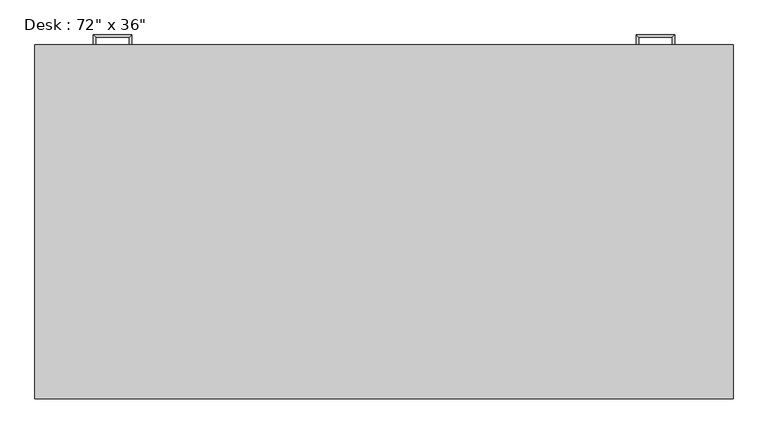
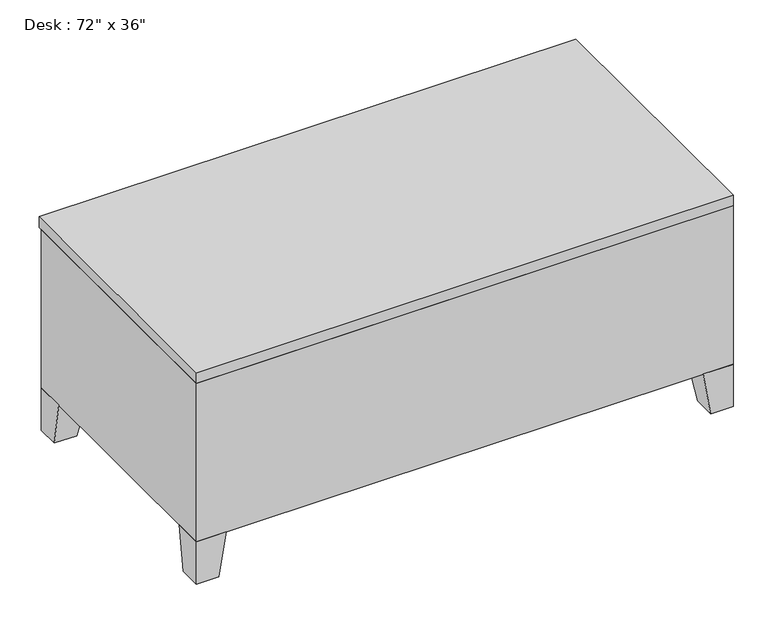
"""IFC4 building model written with IfcOpenShell, lengths in millimetres: furniture geometry."""

import ifcopenshell
import ifcopenshell.guid

model = None  # the IFC model being written
_history = None  # IfcOwnerHistory: only IFC2X3 demands one
_inside = {}  # id of a spatial element -> (the spatial element, [elements in it])
_under = {}  # id of a project, library or spatial element -> (it, [spatial elements below it])
_declared = {}  # id of a project -> (the project, [libraries it declares])
_typed = {}  # id of a type object -> (the type object, [elements of that type])
_made_of = {}  # id of a material, layer set ... -> (it, [elements and type objects made of it])


def new_model(schema):
    """Start an empty IFC model of exactly this schema.

    Asked for "IFC4X3", IfcOpenShell would pick the latest addendum, in which some entities
    have other attributes; the version numbers below select the first issue.
    IFC2X3 requires an IfcOwnerHistory on every rooted entity: one is made here for all.
    """
    global model, _history
    if schema == "IFC4X3":
        model = ifcopenshell.file(schema_version=(4, 3, 0, 0))
    else:
        model = ifcopenshell.file(schema=schema)
    _inside.clear()
    _under.clear()
    _declared.clear()
    _typed.clear()
    _made_of.clear()
    _history = None
    if model.schema == "IFC2X3":
        org = make("IfcOrganization", Name="unknown")
        user = make(
            "IfcPersonAndOrganization",
            ThePerson=make("IfcPerson", FamilyName="unknown"),
            TheOrganization=org,
        )
        app = make(
            "IfcApplication",
            ApplicationDeveloper=org,
            Version="unknown",
            ApplicationFullName="unknown",
            ApplicationIdentifier="unknown",
        )
        _history = make(
            "IfcOwnerHistory",
            OwningUser=user,
            OwningApplication=app,
            ChangeAction="ADDED",
            CreationDate=0,
        )
    return model


def make(cls, **values):
    """One entity of the class cls with the attributes given. An attribute that is None is left unset."""
    return model.create_entity(
        cls, **{name: value for name, value in values.items() if value is not None}
    )


def rooted(cls, **values):
    """An entity with a GlobalId (a new one), such as an element, a storey or a relation."""
    return make(cls, GlobalId=ifcopenshell.guid.new(), OwnerHistory=_history, **values)


def si_unit(unit_type, name, prefix=None):
    """IfcSIUnit, for example si_unit("LENGTHUNIT", "METRE", prefix="MILLI")."""
    return make("IfcSIUnit", UnitType=unit_type, Prefix=prefix, Name=name)


def assignment(units):
    """IfcUnitAssignment: the units of a project."""
    return None if units is None else make("IfcUnitAssignment", Units=units)


def point(xyz):
    """IfcCartesianPoint."""
    return None if xyz is None else make("IfcCartesianPoint", Coordinates=xyz)


def direction(xyz):
    """IfcDirection."""
    return None if xyz is None else make("IfcDirection", DirectionRatios=xyz)


def frame(location, z_axis=None, x_axis=None):
    """IfcAxis2Placement3D, a coordinate frame: its origin and axes. An axis left out is left unset."""
    return make(
        "IfcAxis2Placement3D",
        Location=point(location),
        Axis=direction(z_axis),
        RefDirection=direction(x_axis),
    )


def origin():
    """The frame at (0, 0, 0) with its axes left unset."""
    return frame((0.0, 0.0, 0.0))


def place(relative_to, where):
    """IfcLocalPlacement: puts the frame where relative to a parent placement (None: the world)."""
    return make(
        "IfcLocalPlacement", PlacementRelTo=relative_to, RelativePlacement=where
    )


def context(
    kind, dimensions, precision=None, world=None, true_north=None, identifier=None
):
    """IfcGeometricRepresentationContext, for example the 3D "Model" context."""
    return make(
        "IfcGeometricRepresentationContext",
        ContextIdentifier=identifier,
        ContextType=kind,
        CoordinateSpaceDimension=dimensions,
        Precision=precision,
        WorldCoordinateSystem=world,
        TrueNorth=true_north,
    )


def project(units=None, contexts=None):
    """IfcProject with its units and contexts."""
    return rooted(
        "IfcProject",
        Name="project",
        RepresentationContexts=contexts,
        UnitsInContext=assignment(units),
    )


def spatial(cls, under=None, at=None, **own):
    """A site, building, storey or space (cls), placed at a placement, below another one or the project."""
    s = rooted(cls, ObjectPlacement=at, **own)
    if under is not None:
        _under.setdefault(under.id(), (under, []))[1].append(s)
    return s


def polyline(points):
    """IfcPolyline through the points."""
    return make("IfcPolyline", Points=[point(p) for p in points])


def outline(outer, holes=None, kind="AREA"):
    """IfcArbitraryClosedProfileDef: a profile drawn as a closed curve; with holes, ...WithVoids."""
    if holes is None:
        return make("IfcArbitraryClosedProfileDef", ProfileType=kind, OuterCurve=outer)
    return make(
        "IfcArbitraryProfileDefWithVoids",
        ProfileType=kind,
        OuterCurve=outer,
        InnerCurves=holes,
    )


def extrude(swept, where, along, depth):
    """IfcExtrudedAreaSolid: the profile swept, set in the frame where, extruded along a direction by depth."""
    return make(
        "IfcExtrudedAreaSolid",
        SweptArea=swept,
        Position=where,
        ExtrudedDirection=direction(along),
        Depth=depth,
    )


def faces_of(points, faces, orient=None, outer=None):
    """IfcFace entities. A face is a list of loops; a loop is a list of indices into points, from 0.

    orient and outer hold one flag for each loop. By default every Orientation is true, the
    first loop of a face is its IfcFaceOuterBound and the others are IfcFaceBound.
    """
    made = []
    for i, loops in enumerate(faces):
        bounds = []
        for j, loop in enumerate(loops):
            is_outer = j == 0 if outer is None else outer[i][j]
            bounds.append(
                make(
                    "IfcFaceOuterBound" if is_outer else "IfcFaceBound",
                    Bound=make("IfcPolyLoop", Polygon=[points[k] for k in loop]),
                    Orientation=True if orient is None else orient[i][j],
                )
            )
        made.append(make("IfcFace", Bounds=bounds))
    return made


def faceted_brep(points, faces, orient=None, outer=None, voids=None):
    """IfcFacetedBrep: a solid bounded by flat faces; with voids (closed shells), ...WithVoids."""
    shared = [point(p) for p in points]
    hull = make("IfcClosedShell", CfsFaces=faces_of(shared, faces, orient, outer))
    if voids is None:
        return make("IfcFacetedBrep", Outer=hull)
    return make(
        "IfcFacetedBrepWithVoids",
        Outer=hull,
        Voids=[
            make(cls, CfsFaces=faces_of(shared, fs, o, b)) for cls, fs, o, b in voids
        ],
    )


def shape(context_of_items, identifier, shape_type, items):
    """IfcShapeRepresentation: the items that make up one representation, for example the "Body"."""
    return make(
        "IfcShapeRepresentation",
        ContextOfItems=context_of_items,
        RepresentationIdentifier=identifier,
        RepresentationType=shape_type,
        Items=items,
    )


def source(mapping_origin, context_of_items, identifier, shape_type, items):
    """IfcRepresentationMap: a shape defined once, which mapped items show again and again."""
    return make(
        "IfcRepresentationMap",
        MappingOrigin=mapping_origin,
        MappedRepresentation=shape(context_of_items, identifier, shape_type, items),
    )


def transform(
    local_origin,
    x_axis=None,
    y_axis=None,
    z_axis=None,
    scale=None,
    scale2=None,
    scale3=None,
    uniform=True,
):
    """IfcCartesianTransformationOperator3D, or its non-uniform kind. x_axis, y_axis, z_axis: its Axis1, 2, 3."""
    if uniform:
        return make(
            "IfcCartesianTransformationOperator3D",
            Axis1=direction(x_axis),
            Axis2=direction(y_axis),
            LocalOrigin=point(local_origin),
            Scale=scale,
            Axis3=direction(z_axis),
        )
    return make(
        "IfcCartesianTransformationOperator3DnonUniform",
        Axis1=direction(x_axis),
        Axis2=direction(y_axis),
        LocalOrigin=point(local_origin),
        Scale=scale,
        Axis3=direction(z_axis),
        Scale2=scale2,
        Scale3=scale3,
    )


def mapped(mapping_source, mapping_target):
    """IfcMappedItem: shows the shape of a source again, moved by a transform."""
    return make(
        "IfcMappedItem", MappingSource=mapping_source, MappingTarget=mapping_target
    )


def made_of(thing, what):
    """Note that an element or type object is made of a material, layer set ...; save() writes the relation."""
    if what is not None:
        _made_of.setdefault(what.id(), (what, []))[1].append(thing)
    return thing


def element(
    cls,
    number,
    at=None,
    inside=None,
    cuts=None,
    type_object=None,
    material=None,
    context=None,
    identifier="Body",
    shape_type=None,
    held_by="IfcProductDefinitionShape",
    body=None,
    shapes=None,
    **own,
):
    """One element of the class cls, such as IfcWall. Its Tag is "e" and its number.

    at: its placement. inside: the storey or other place that contains it. cuts: it is an
    opening in that element (IfcRelVoidsElement). A single representation is given by context,
    identifier, shape_type and body (its items); several are given by shapes. held_by: the class
    of the entity that holds the representations. save() writes the other relations.
    """
    e = rooted(cls, Tag="e%d" % number, ObjectPlacement=at, **own)
    if body is not None:
        shapes = [shape(context, identifier, shape_type, body)]
    if shapes is not None:
        e.Representation = make(held_by, Representations=shapes)
    if inside is not None:
        _inside.setdefault(inside.id(), (inside, []))[1].append(e)
    if cuts is not None:
        rooted(
            "IfcRelVoidsElement", RelatingBuildingElement=cuts, RelatedOpeningElement=e
        )
    if type_object is not None:
        _typed.setdefault(type_object.id(), (type_object, []))[1].append(e)
    return made_of(e, material)


def aggregate(whole, parts):
    """IfcRelAggregates: a whole, such as a stair, and the parts it consists of."""
    return rooted("IfcRelAggregates", RelatingObject=whole, RelatedObjects=parts)


def save(model, path):
    """Write the relations noted so far, then the file.

    IfcRelAggregates (storeys below a building ...), IfcRelContainedInSpatialStructure (elements
    in a storey), IfcRelDefinesByType, IfcRelAssociatesMaterial and IfcRelDeclares: one each for
    every whole, place, type object, material and project.
    """
    for whole, parts in _under.values():
        aggregate(whole, parts)
    for where, things in _inside.values():
        rooted(
            "IfcRelContainedInSpatialStructure",
            RelatedElements=things,
            RelatingStructure=where,
        )
    for kind, things in _typed.values():
        rooted("IfcRelDefinesByType", RelatedObjects=things, RelatingType=kind)
    for what, things in _made_of.values():
        rooted("IfcRelAssociatesMaterial", RelatedObjects=things, RelatingMaterial=what)
    for by, libraries in _declared.values():
        rooted("IfcRelDeclares", RelatingContext=by, RelatedDefinitions=libraries)
    model.write(path)


def furniture_65204735(model_context):
    return source(origin(), model_context, "Body", "SolidModel", [
        extrude(outline(polyline([(-133.35, 76.2), (-133.35, 88.9), (234.95, 88.9), (234.95, 76.2), (-133.35, 76.2)])), frame((0.0, 0.0, 603.25), z_axis=(0.0, 0.0, 1.0), x_axis=(1.0, 0.0, 0.0)), (0.0, 0.0, 1.0), 101.6),
        extrude(outline(polyline([(-133.35, 76.2), (-133.35, 88.9), (234.95, 88.9), (234.95, 76.2), (-133.35, 76.2)])), frame((0.0, 0.0, 171.45), z_axis=(0.0, 0.0, 1.0), x_axis=(1.0, 0.0, 0.0)), (0.0, 0.0, 1.0), 412.75),
        extrude(outline(polyline([(1289.05, 76.2), (1289.05, 88.9), (1657.35, 88.9), (1657.35, 76.2), (1289.05, 76.2)])), frame((0.0, 0.0, 603.25), z_axis=(0.0, 0.0, 1.0), x_axis=(1.0, 0.0, 0.0)), (0.0, 0.0, 1.0), 101.6),
        extrude(outline(polyline([(1289.05, 76.2), (1289.05, 88.9), (1657.35, 88.9), (1657.35, 76.2), (1289.05, 76.2)])), frame((0.0, 0.0, 171.45), z_axis=(0.0, 0.0, 1.0), x_axis=(1.0, 0.0, 0.0)), (0.0, 0.0, 1.0), 171.45),
        extrude(outline(polyline([(1289.05, 76.2), (1289.05, 88.9), (1657.35, 88.9), (1657.35, 76.2), (1289.05, 76.2)])), frame((0.0, 0.0, 482.6), z_axis=(0.0, 0.0, 1.0), x_axis=(1.0, 0.0, 0.0)), (0.0, 0.0, 1.0), 101.6),
        extrude(outline(polyline([(1289.05, 76.2), (1289.05, 88.9), (1657.35, 88.9), (1657.35, 76.2), (1289.05, 76.2)])), frame((0.0, 0.0, 361.95), z_axis=(0.0, 0.0, 1.0), x_axis=(1.0, 0.0, 0.0)), (0.0, 0.0, 1.0), 101.6),
        faceted_brep([(-50.8, 76.2, 152.4), (-152.4, 76.2, 152.4), (-152.4, -25.4, 152.4), (-50.8, -25.4, 152.4), (-76.2, 76.2, 0.0), (-76.2, 0.0, 0.0), (-152.4, 0.0, 0.0), (-152.4, 76.2, 0.0)], [[[0, 1, 2, 3]], [[4, 5, 6, 7]], [[4, 0, 3, 5]], [[5, 3, 2, 6]], [[6, 2, 1, 7]], [[7, 1, 0, 4]]]),
        faceted_brep([(-50.8, -838.2, 152.4), (-50.8, -736.6, 152.4), (-152.4, -736.6, 152.4), (-152.4, -838.2, 152.4), (-76.2, -838.2, 0.0), (-152.4, -838.2, 0.0), (-152.4, -762.0, 0.0), (-76.2, -762.0, 0.0)], [[[0, 1, 2, 3]], [[4, 5, 6, 7]], [[4, 0, 3, 5]], [[5, 3, 2, 6]], [[6, 2, 1, 7]], [[7, 1, 0, 4]]]),
        faceted_brep([(1574.8, -838.2, 152.4), (1676.4, -838.2, 152.4), (1676.4, -736.6, 152.4), (1574.8, -736.6, 152.4), (1600.2, -838.2, 0.0), (1600.2, -762.0, 0.0), (1676.4, -762.0, 0.0), (1676.4, -838.2, 0.0)], [[[0, 1, 2, 3]], [[4, 5, 6, 7]], [[4, 0, 3, 5]], [[5, 3, 2, 6]], [[6, 2, 1, 7]], [[7, 1, 0, 4]]]),
        faceted_brep([(1574.8, 76.2, 152.4), (1574.8, -25.4, 152.4), (1676.4, -25.4, 152.4), (1676.4, 76.2, 152.4), (1600.2, 76.2, 0.0), (1676.4, 76.2, 0.0), (1676.4, 0.0, 0.0), (1600.2, 0.0, 0.0)], [[[0, 1, 2, 3]], [[4, 5, 6, 7]], [[4, 0, 3, 5]], [[5, 3, 2, 6]], [[6, 2, 1, 7]], [[7, 1, 0, 4]]]),
        extrude(outline(polyline([(-152.4, 88.9), (1676.4, 88.9), (1676.4, -838.2), (-152.4, -838.2), (-152.4, 88.9)])), frame((0.0, 0.0, 723.9), z_axis=(0.0, 0.0, 1.0), x_axis=(1.0, 0.0, 0.0)), (0.0, 0.0, 1.0), 38.1),
        extrude(outline(polyline([(1270.0, 76.2), (1676.4, 76.2), (1676.4, -838.2), (-152.4, -838.2), (-152.4, 76.2), (254.0, 76.2), (254.0, -711.2), (1270.0, -711.2), (1270.0, 76.2)])), frame((0.0, 0.0, 152.4), z_axis=(0.0, 0.0, 1.0), x_axis=(1.0, 0.0, 0.0)), (0.0, 0.0, 1.0), 571.5),
        faceted_brep([(6.35, 88.9, 546.1), (0.0, 88.9, 546.1), (0.0, 88.9, 533.4), (6.35, 88.9, 533.4), (6.35, 107.95, 533.4), (6.35, 107.95, 546.1), (0.0, 114.3, 533.4), (0.0, 114.3, 546.1), (95.25, 107.95, 533.4), (95.25, 107.95, 546.1), (101.6, 114.3, 533.4), (101.6, 114.3, 546.1), (95.25, 88.9, 546.1), (95.25, 88.9, 533.4), (101.6, 88.9, 533.4), (101.6, 88.9, 546.1)], [[[0, 1, 2, 3]], [[3, 4, 5, 0]], [[2, 6, 4, 3]], [[1, 7, 6, 2]], [[0, 5, 7, 1]], [[4, 8, 9, 5]], [[6, 10, 8, 4]], [[7, 11, 10, 6]], [[5, 9, 11, 7]], [[12, 13, 14, 15]], [[8, 13, 12, 9]], [[10, 14, 13, 8]], [[11, 15, 14, 10]], [[9, 12, 15, 11]]]),
        faceted_brep([(6.35, 88.9, 666.75), (0.0, 88.9, 666.75), (0.0, 88.9, 654.05), (6.35, 88.9, 654.05), (6.35, 107.95, 654.05), (6.35, 107.95, 666.75), (0.0, 114.3, 654.05), (0.0, 114.3, 666.75), (95.25, 107.95, 654.05), (95.25, 107.95, 666.75), (101.6, 114.3, 654.05), (101.6, 114.3, 666.75), (95.25, 88.9, 666.75), (95.25, 88.9, 654.05), (101.6, 88.9, 654.05), (101.6, 88.9, 666.75)], [[[0, 1, 2, 3]], [[3, 4, 5, 0]], [[2, 6, 4, 3]], [[1, 7, 6, 2]], [[0, 5, 7, 1]], [[4, 8, 9, 5]], [[6, 10, 8, 4]], [[7, 11, 10, 6]], [[5, 9, 11, 7]], [[12, 13, 14, 15]], [[8, 13, 12, 9]], [[10, 14, 13, 8]], [[11, 15, 14, 10]], [[9, 12, 15, 11]]]),
        faceted_brep([(1517.65, 88.9, 304.8), (1517.65, 88.9, 292.1), (1524.0, 88.9, 292.1), (1524.0, 88.9, 304.8), (1524.0, 114.3, 304.8), (1517.65, 107.95, 304.8), (1524.0, 114.3, 292.1), (1517.65, 107.95, 292.1), (1422.4, 114.3, 304.8), (1428.75, 107.95, 304.8), (1422.4, 114.3, 292.1), (1428.75, 107.95, 292.1), (1428.75, 88.9, 304.8), (1422.4, 88.9, 304.8), (1422.4, 88.9, 292.1), (1428.75, 88.9, 292.1)], [[[0, 1, 2, 3]], [[3, 4, 5, 0]], [[2, 6, 4, 3]], [[1, 7, 6, 2]], [[0, 5, 7, 1]], [[4, 8, 9, 5]], [[6, 10, 8, 4]], [[7, 11, 10, 6]], [[5, 9, 11, 7]], [[12, 13, 14, 15]], [[8, 13, 12, 9]], [[10, 14, 13, 8]], [[11, 15, 14, 10]], [[9, 12, 15, 11]]]),
        faceted_brep([(1517.65, 88.9, 425.45), (1517.65, 88.9, 412.75), (1524.0, 88.9, 412.75), (1524.0, 88.9, 425.45), (1524.0, 114.3, 425.45), (1517.65, 107.95, 425.45), (1524.0, 114.3, 412.75), (1517.65, 107.95, 412.75), (1422.4, 114.3, 425.45), (1428.75, 107.95, 425.45), (1422.4, 114.3, 412.75), (1428.75, 107.95, 412.75), (1428.75, 88.9, 425.45), (1422.4, 88.9, 425.45), (1422.4, 88.9, 412.75), (1428.75, 88.9, 412.75)], [[[0, 1, 2, 3]], [[3, 4, 5, 0]], [[2, 6, 4, 3]], [[1, 7, 6, 2]], [[0, 5, 7, 1]], [[4, 8, 9, 5]], [[6, 10, 8, 4]], [[7, 11, 10, 6]], [[5, 9, 11, 7]], [[12, 13, 14, 15]], [[8, 13, 12, 9]], [[10, 14, 13, 8]], [[11, 15, 14, 10]], [[9, 12, 15, 11]]]),
        faceted_brep([(1517.65, 88.9, 546.1), (1517.65, 88.9, 533.4), (1524.0, 88.9, 533.4), (1524.0, 88.9, 546.1), (1524.0, 114.3, 546.1), (1517.65, 107.95, 546.1), (1524.0, 114.3, 533.4), (1517.65, 107.95, 533.4), (1422.4, 114.3, 546.1), (1428.75, 107.95, 546.1), (1422.4, 114.3, 533.4), (1428.75, 107.95, 533.4), (1428.75, 88.9, 546.1), (1422.4, 88.9, 546.1), (1422.4, 88.9, 533.4), (1428.75, 88.9, 533.4)], [[[0, 1, 2, 3]], [[3, 4, 5, 0]], [[2, 6, 4, 3]], [[1, 7, 6, 2]], [[0, 5, 7, 1]], [[4, 8, 9, 5]], [[6, 10, 8, 4]], [[7, 11, 10, 6]], [[5, 9, 11, 7]], [[12, 13, 14, 15]], [[8, 13, 12, 9]], [[10, 14, 13, 8]], [[11, 15, 14, 10]], [[9, 12, 15, 11]]]),
        faceted_brep([(1517.65, 88.9, 666.75), (1517.65, 88.9, 654.05), (1524.0, 88.9, 654.05), (1524.0, 88.9, 666.75), (1524.0, 114.3, 666.75), (1517.65, 107.95, 666.75), (1524.0, 114.3, 654.05), (1517.65, 107.95, 654.05), (1422.4, 114.3, 666.75), (1428.75, 107.95, 666.75), (1422.4, 114.3, 654.05), (1428.75, 107.95, 654.05), (1428.75, 88.9, 666.75), (1422.4, 88.9, 666.75), (1422.4, 88.9, 654.05), (1428.75, 88.9, 654.05)], [[[0, 1, 2, 3]], [[3, 4, 5, 0]], [[2, 6, 4, 3]], [[1, 7, 6, 2]], [[0, 5, 7, 1]], [[4, 8, 9, 5]], [[6, 10, 8, 4]], [[7, 11, 10, 6]], [[5, 9, 11, 7]], [[12, 13, 14, 15]], [[8, 13, 12, 9]], [[10, 14, 13, 8]], [[11, 15, 14, 10]], [[9, 12, 15, 11]]]),
    ])


if __name__ == "__main__":
    model = new_model("IFC4")
    model_context = context("Model", 3, world=origin())
    ifc_project = project(units=[si_unit("LENGTHUNIT", "METRE", prefix="MILLI")], contexts=[model_context])
    site = spatial("IfcSite", under=ifc_project)
    building = spatial("IfcBuilding", under=site)
    placement = place(None, origin())
    furniture_shape = furniture_65204735(model_context)
    element("IfcFurniture", 1, ObjectType="Desk : 72\" x 36\"", at=placement, inside=building, context=model_context, shape_type="MappedRepresentation", body=[
        mapped(furniture_shape, transform((0.0, 0.0, 0.0), x_axis=(1.0, 0.0, 0.0), y_axis=(0.0, 1.0, 0.0), z_axis=(0.0, 0.0, 1.0))),
    ])
    save(model, "model.ifc")

# Revit data of these elements
# Type "Desk : 72\" x 36\""
#   Assembly Code = "E2020200"
#   Depth = 3' - 0"
#   Height = 2' - 6"
#   Leg Height = 0' - 6"
#   Width = 6' - 0"
#   Body Material = Laminate, Ivory, Matte
#   Handle/Leg Material = Steel, Chrome Plated
#   Top Material = Cherry
#   Default Elevation = 0
# Element 1 (IfcFurniture, "Desk : 72\" x 36\"")
#   Materials on its faces: "Steel, Chrome Plated", "Laminate, Ivory, Matte", "Cherry"
# Materials
#   "Laminate, Ivory, Matte": class "Plastic", colour RGB 247 247 239, transparency 0, Description = "Plastic Laminate - Ivory, Matte", Cost = 0
#   "Steel, Chrome Plated": class "Metal", colour RGB 17 17 17, transparency 0, Description = "Chromiuim plated steel", Cost = 0
#   "Cherry": class "Wood", colour RGB 226 177 128, transparency 0, Description = "Prunus Serotina", Cost = 0
